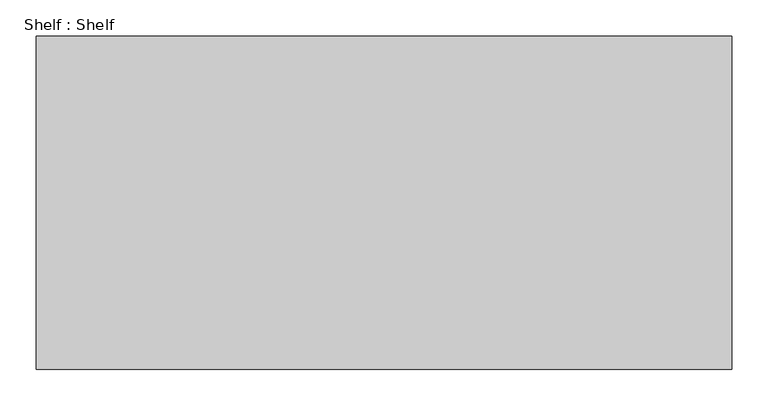
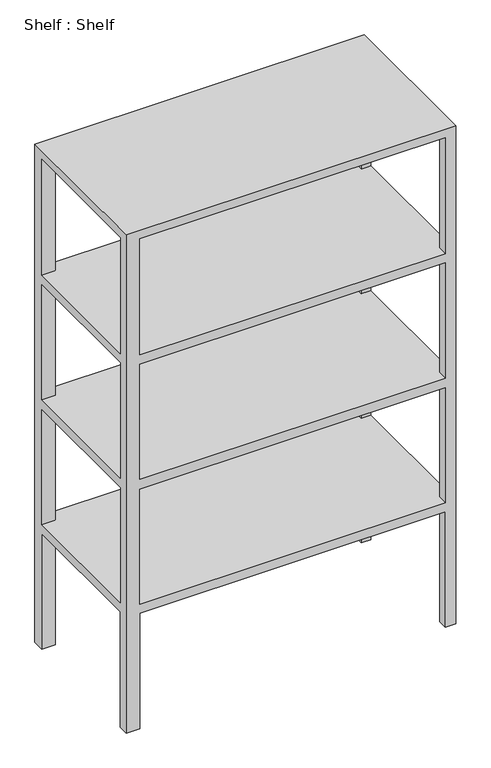
"""IFC4 building model written with IfcOpenShell, lengths in millimetres: furniture geometry, Shelf : Shelf."""

from ifc_helpers import new_model, si_unit, origin, place, context, project, spatial, faceted_brep, source, transform, mapped, element, save


def shelf_shelf_d39eace1(model_context):
    return source(origin(), model_context, "Body", "Brep", [
        faceted_brep([(14056.7001442, 3277.8615366, 1524.0), (13103.4798744, 3277.8615366, 1524.0), (13103.4798744, 2820.6615366, 1524.0), (14056.7001442, 2820.6615366, 1524.0), (14056.7001442, 2849.585331, 0.0), (14056.7001442, 2820.6615366, 0.0), (14027.0281946, 2820.6615366, 0.0), (14027.0281946, 2849.585331, 0.0), (14056.7001442, 3277.8615366, 0.0), (14056.7001442, 3245.3048936, 0.0), (14028.3529362, 3245.3048936, 0.0), (14028.3529362, 3277.8615366, 0.0), (13142.3001442, 2820.6615366, 0.0), (13103.4798744, 2820.6615366, 0.0), (13103.4798744, 2849.585331, 0.0), (13142.3001442, 2849.585331, 0.0), (13103.4798744, 3244.0675604, 0.0), (13103.4798744, 3277.8615366, 0.0), (13142.3001442, 3277.8615366, 0.0), (13142.3001442, 3244.0675604, 0.0), (14028.3529362, 3277.8615366, 353.3332002), (13142.3001442, 3277.8615366, 353.3332002), (14028.3529362, 3277.8615366, 1497.6781444), (13142.3001442, 3277.8615366, 1497.6781444), (13142.3001442, 3277.8615366, 1143.0), (14028.3529362, 3277.8615366, 1143.0), (14028.3529362, 3277.8615366, 1114.8196695), (13142.3001442, 3277.8615366, 1114.8196695), (13142.3001442, 3277.8615366, 762.0), (14028.3529362, 3277.8615366, 762.0), (14028.3529362, 3277.8615366, 731.9611947), (13142.3001442, 3277.8615366, 731.9611947), (13142.3001442, 3277.8615366, 381.0), (14028.3529362, 3277.8615366, 381.0), (13103.4798744, 3244.0675604, 353.3332002), (13103.4798744, 2849.585331, 353.3332002), (13103.4798744, 3244.0675604, 1497.6781444), (13103.4798744, 2849.585331, 1497.6781444), (13103.4798744, 2849.585331, 1143.0), (13103.4798744, 3244.0675604, 1143.0), (13103.4798744, 3244.0675604, 1114.8196695), (13103.4798744, 2849.585331, 1114.8196695), (13103.4798744, 2849.585331, 762.0), (13103.4798744, 3244.0675604, 762.0), (13103.4798744, 3244.0675604, 731.9611947), (13103.4798744, 2849.585331, 731.9611947), (13103.4798744, 2849.585331, 381.0), (13103.4798744, 3244.0675604, 381.0), (13142.3001442, 2820.6615366, 353.3332002), (14027.0281946, 2820.6615366, 353.3332002), (13142.3001442, 2820.6615366, 1497.6781444), (14027.0281946, 2820.6615366, 1497.6781444), (14027.0281946, 2820.6615366, 1143.0), (13142.3001442, 2820.6615366, 1143.0), (13142.3001442, 2820.6615366, 1114.8196695), (14027.0281946, 2820.6615366, 1114.8196695), (14027.0281946, 2820.6615366, 762.0), (13142.3001442, 2820.6615366, 762.0), (13142.3001442, 2820.6615366, 731.9611947), (14027.0281946, 2820.6615366, 731.9611947), (14027.0281946, 2820.6615366, 381.0), (13142.3001442, 2820.6615366, 381.0), (14056.7001442, 2849.585331, 353.3332002), (14056.7001442, 3245.3048936, 353.3332002), (14056.7001442, 2849.585331, 1497.6781444), (14056.7001442, 3245.3048936, 1497.6781444), (14056.7001442, 3245.3048936, 1143.0), (14056.7001442, 2849.585331, 1143.0), (14056.7001442, 2849.585331, 1114.8196695), (14056.7001442, 3245.3048936, 1114.8196695), (14056.7001442, 3245.3048936, 762.0), (14056.7001442, 2849.585331, 762.0), (14056.7001442, 2849.585331, 731.9611947), (14056.7001442, 3245.3048936, 731.9611947), (14056.7001442, 3245.3048936, 381.0), (14056.7001442, 2849.585331, 381.0), (13142.3001442, 2849.585331, 1497.6781444), (13142.3001442, 3244.0675604, 1497.6781444), (14028.3529362, 3245.3048936, 1497.6781444), (14027.0281946, 2849.585331, 1497.6781444), (13142.3001442, 2849.585331, 1143.0), (14027.0281946, 2849.585331, 1143.0), (14028.3529362, 3245.3048936, 1143.0), (13142.3001442, 3244.0675604, 1143.0), (13142.3001442, 2849.585331, 1114.8196695), (13142.3001442, 3244.0675604, 1114.8196695), (14028.3529362, 3245.3048936, 1114.8196695), (14027.0281946, 2849.585331, 1114.8196695), (13142.3001442, 2849.585331, 762.0), (14027.0281946, 2849.585331, 762.0), (14028.3529362, 3245.3048936, 762.0), (13142.3001442, 3244.0675604, 762.0), (13142.3001442, 2849.585331, 731.9611947), (13142.3001442, 3244.0675604, 731.9611947), (14028.3529362, 3245.3048936, 731.9611947), (14027.0281946, 2849.585331, 731.9611947), (13142.3001442, 2849.585331, 381.0), (14027.0281946, 2849.585331, 381.0), (14028.3529362, 3245.3048936, 381.0), (13142.3001442, 3244.0675604, 381.0), (13142.3001442, 2849.585331, 353.3332002), (13142.3001442, 3244.0675604, 353.3332002), (14028.3529362, 3245.3048936, 353.3332002), (14027.0281946, 2849.585331, 353.3332002)], [[[0, 1, 2, 3]], [[4, 5, 6, 7]], [[8, 9, 10, 11]], [[12, 13, 14, 15]], [[16, 17, 18, 19]], [[1, 0, 8, 11, 20, 21, 18, 17], [22, 23, 24, 25], [26, 27, 28, 29], [30, 31, 32, 33]], [[2, 1, 17, 16, 34, 35, 14, 13], [36, 37, 38, 39], [40, 41, 42, 43], [44, 45, 46, 47]], [[3, 2, 13, 12, 48, 49, 6, 5], [50, 51, 52, 53], [54, 55, 56, 57], [58, 59, 60, 61]], [[0, 3, 5, 4, 62, 63, 9, 8], [64, 65, 66, 67], [68, 69, 70, 71], [72, 73, 74, 75]], [[76, 37, 36, 77, 23, 22, 78, 65, 64, 79, 51, 50]], [[80, 53, 52, 81, 67, 66, 82, 25, 24, 83, 39, 38]], [[76, 50, 53, 80]], [[51, 79, 81, 52]], [[79, 64, 67, 81]], [[65, 78, 82, 66]], [[78, 22, 25, 82]], [[23, 77, 83, 24]], [[77, 36, 39, 83]], [[37, 76, 80, 38]], [[84, 41, 40, 85, 27, 26, 86, 69, 68, 87, 55, 54]], [[88, 57, 56, 89, 71, 70, 90, 29, 28, 91, 43, 42]], [[84, 54, 57, 88]], [[55, 87, 89, 56]], [[87, 68, 71, 89]], [[69, 86, 90, 70]], [[86, 26, 29, 90]], [[27, 85, 91, 28]], [[85, 40, 43, 91]], [[41, 84, 88, 42]], [[92, 45, 44, 93, 31, 30, 94, 73, 72, 95, 59, 58]], [[96, 61, 60, 97, 75, 74, 98, 33, 32, 99, 47, 46]], [[92, 58, 61, 96]], [[59, 95, 97, 60]], [[95, 72, 75, 97]], [[73, 94, 98, 74]], [[94, 30, 33, 98]], [[31, 93, 99, 32]], [[93, 44, 47, 99]], [[45, 92, 96, 46]], [[100, 35, 34, 101, 21, 20, 102, 63, 62, 103, 49, 48]], [[100, 48, 12, 15]], [[49, 103, 7, 6]], [[103, 62, 4, 7]], [[63, 102, 10, 9]], [[102, 20, 11, 10]], [[21, 101, 19, 18]], [[101, 34, 16, 19]], [[35, 100, 15, 14]]]),
    ])


if __name__ == "__main__":
    model = new_model("IFC4")
    model_context = context("Model", 3, world=origin())
    ifc_project = project(units=[si_unit("LENGTHUNIT", "METRE", prefix="MILLI")], contexts=[model_context])
    site = spatial("IfcSite", under=ifc_project)
    building = spatial("IfcBuilding", under=site)
    placement = place(None, origin())
    shelf_shelf_shape = shelf_shelf_d39eace1(model_context)
    element("IfcFurniture", 1, ObjectType="Shelf : Shelf", at=placement, inside=building, context=model_context, shape_type="MappedRepresentation", body=[
        mapped(shelf_shelf_shape, transform((0.0, 0.0, 0.0), x_axis=(1.0, 0.0, 0.0), y_axis=(0.0, 1.0, 0.0), z_axis=(0.0, 0.0, 1.0))),
    ])
    save(model, "model.ifc")

# Revit data of these elements
# Element 1 (IfcFurniture, "Shelf : Shelf")
#   Materials on its faces: "food"
# Materials
#   "food": class "Glass", colour RGB 233 233 233, transparency 0, Description = "Soda Lime Glass", Cost = 0
